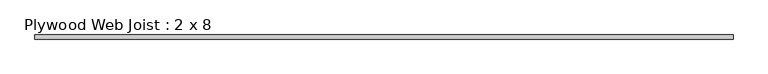
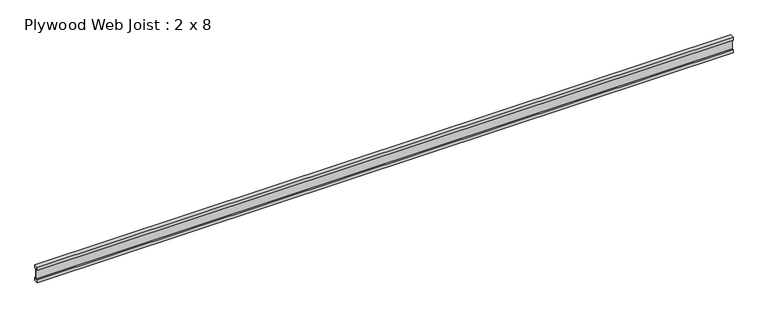
"""IFC4 building model written with IfcOpenShell, lengths in millimetres: beam geometry, Plywood Web Joist : 2 x 8."""

from ifc_helpers import new_model, si_unit, frame, origin, place, context, project, spatial, polyline, outline, extrude, source, transform, mapped, element, save


def plywood_web_joist_2_x_8_7c958bd9(model_context):
    return source(origin(), model_context, "Body", "SweptSolid", [
        extrude(outline(polyline([(-25.4, 101.6), (25.4, 101.6), (25.4, 63.5), (4.7625, 63.5), (4.7625, 69.85), (-4.7625, 69.85), (-4.7625, 63.5), (-25.4, 63.5), (-25.4, 101.6)])), frame((-4318.0, 0.0, 0.0), z_axis=(1.0, 0.0, 0.0), x_axis=(0.0, 1.0, 0.0)), (0.0, 0.0, 1.0), 8636.0),
        extrude(outline(polyline([(25.4, -63.5), (25.4, -101.6), (-25.4, -101.6), (-25.4, -63.5), (-4.7625, -63.5), (-4.7625, -69.1160374), (4.7625, -69.1160374), (4.7625, -63.5), (25.4, -63.5)])), frame((-4318.0, 0.0, 0.0), z_axis=(1.0, 0.0, 0.0), x_axis=(0.0, 1.0, 0.0)), (0.0, 0.0, 1.0), 8636.0),
        extrude(outline(polyline([(4318.0, 4.7625), (4318.0, -4.7625), (-4318.0, -4.7625), (-4318.0, 4.7625), (4318.0, 4.7625)])), frame((0.0, 0.0, -69.1160374), z_axis=(0.0, 0.0, 1.0), x_axis=(1.0, 0.0, 0.0)), (0.0, 0.0, 1.0), 138.9660374),
    ])


if __name__ == "__main__":
    model = new_model("IFC4")
    model_context = context("Model", 3, world=origin())
    ifc_project = project(units=[si_unit("LENGTHUNIT", "METRE", prefix="MILLI")], contexts=[model_context])
    site = spatial("IfcSite", under=ifc_project)
    building = spatial("IfcBuilding", under=site)
    placement = place(None, origin())
    plywood_web_joist_2_x_8_shape = plywood_web_joist_2_x_8_7c958bd9(model_context)
    element("IfcBeam", 1, ObjectType="Plywood Web Joist : 2 x 8", at=placement, inside=building, context=model_context, shape_type="MappedRepresentation", body=[
        mapped(plywood_web_joist_2_x_8_shape, transform((0.0, 0.0, 0.0), x_axis=(1.0, 0.0, 0.0), y_axis=(0.0, 1.0, 0.0), z_axis=(0.0, 0.0, 1.0))),
    ])
    save(model, "model.ifc")

# Revit data of these elements
# Type "Plywood Web Joist : 2 x 8"
#   Assembly Code = "B10"
#   Length [instance default] = 5' - 0"
#   b = 0' - 2"
#   d = 0' - 8"
#   Structural Material [instance default] = Softwood, Lumber
# Element 1 (IfcBeam, "Plywood Web Joist : 2 x 8")
#   Materials on its faces: "Softwood, Lumber"
# Materials
#   "Softwood, Lumber": class "Wood", colour RGB 144 113 62, transparency 0, Description = "Pinus Echinata", Cost = 0
